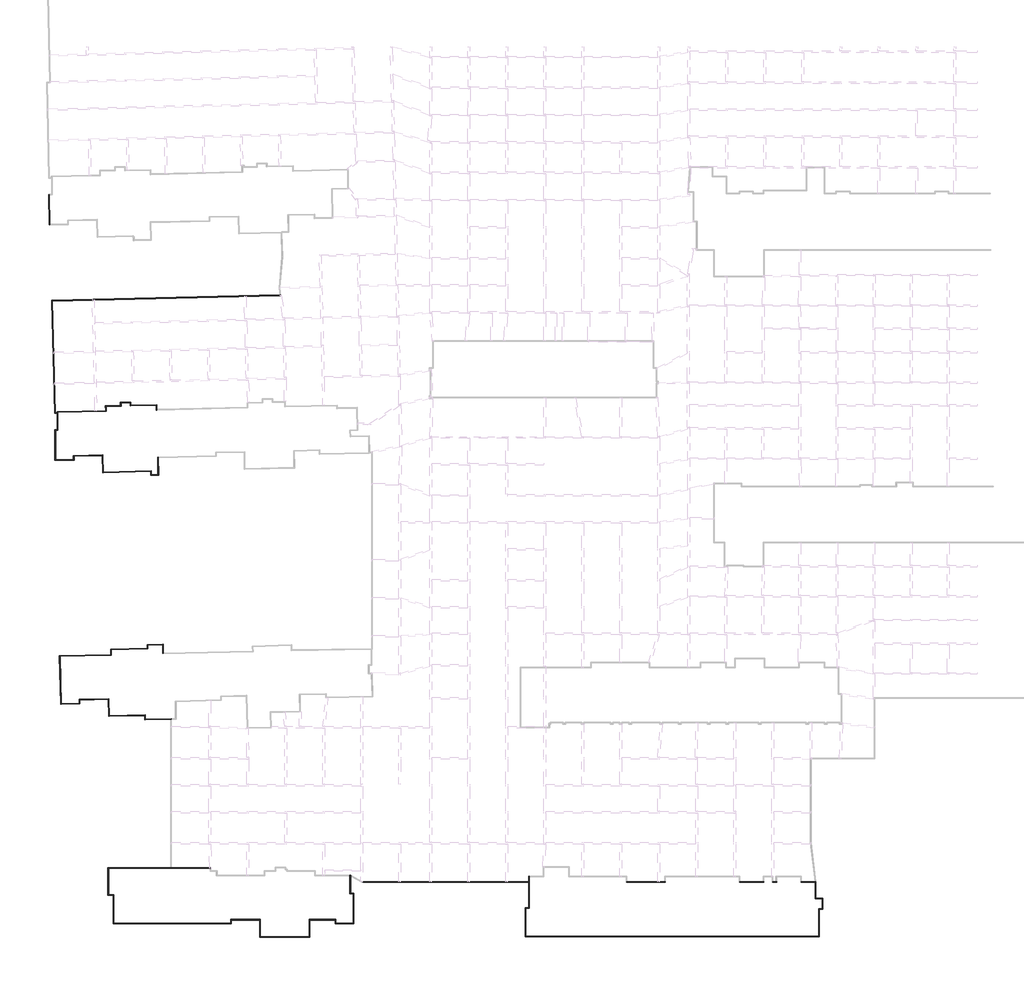
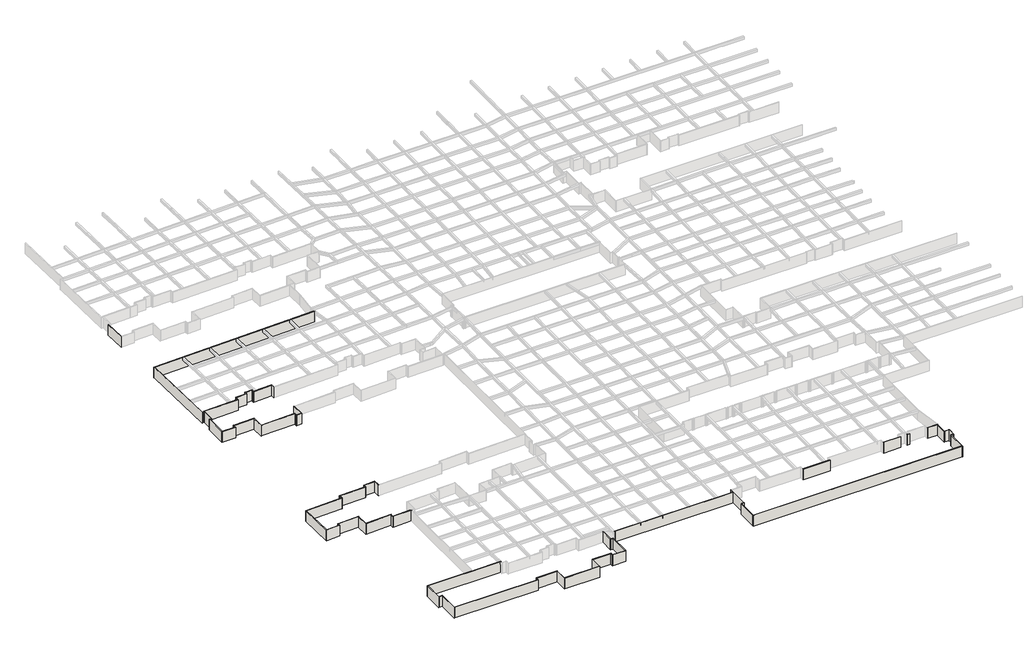
# One storey, part 1 of 20: 68 walls.
"""IFC4 building model written with IfcOpenShell, lengths in millimetres."""

from ifc_helpers import new_model, si_unit, origin, origin_with_axes, place, context, project, spatial, polyline, outline, extrude, faceted_brep, element, save

model = new_model("IFC4")

# Units and contexts
model_context = context("Model", 3, world=origin())
ifc_project = project(units=[si_unit("LENGTHUNIT", "METRE", prefix="MILLI")], contexts=[model_context])

# Site, building, storey
site = spatial("IfcSite", under=ifc_project)
building = spatial("IfcBuilding", under=site)
storey = spatial("IfcBuildingStorey", under=building, Name="户型图", Elevation=0.0)

# Walls
placement = place(None, origin())
element("IfcWall", 1, ObjectType="所有墙体", at=placement, inside=storey, context=model_context, shape_type="Brep", body=[
    faceted_brep([(-25788.9498199, 144552.0423241, 0.0), (-25635.5251271, 138236.5605216, 0.0), (-25635.5251271, 138236.5605216, 3300.0), (-25788.9498199, 144552.0423241, 3300.0), (-25668.9144149, 144552.0423241, 0.0), (-25668.9144149, 144552.0423241, 3300.0), (-25518.4748729, 138359.4394784, 3300.0), (-25515.5605216, 138239.4748729, 3300.0), (-25515.5605216, 138239.4748729, 0.0), (-25518.4748729, 138359.4394784, 0.0)], [[[0, 1, 2, 3]], [[4, 5, 6, 7, 8, 9]], [[1, 0, 4, 9, 8]], [[3, 2, 7, 6, 5]], [[0, 3, 5, 4]], [[2, 1, 8, 7]]]),
])
element("IfcWall", 2, ObjectType="所有墙体", at=placement, inside=storey, context=model_context, shape_type="Brep", body=[
    faceted_brep([(22969.277881, 123512.5246746, 0.0), (-25101.4287529, 122353.5363846, 0.0), (-25101.4287529, 122353.5363846, 3300.0), (22969.277881, 123512.5246746, 3300.0), (22986.0907128, 123392.8951605, 0.0), (22986.0907128, 123392.8951605, 3300.0), (-24978.5712471, 122236.4636154, 3300.0), (-25098.5363846, 122233.5712471, 3300.0), (-25098.5363846, 122233.5712471, 0.0), (-24978.5712471, 122236.4636154, 0.0)], [[[0, 1, 2, 3]], [[4, 5, 6, 7, 8, 9]], [[1, 0, 4, 9, 8]], [[3, 2, 7, 6, 5]], [[0, 3, 5, 4]], [[2, 1, 8, 7]]]),
])
element("IfcWall", 3, ObjectType="所有墙体", at=placement, inside=storey, context=model_context, shape_type="Brep", body=[
    faceted_brep([(-25098.5363846, 122233.5712471, 0.0), (-24529.7383934, 98641.8562998, 0.0), (-24529.7383934, 98641.8562998, 3300.0), (-25098.5363846, 122233.5712471, 3300.0), (-24978.5712471, 122236.4636154, 0.0), (-24978.5712471, 122236.4636154, 3300.0), (-24412.5967296, 98761.8562998, 3300.0), (-24409.7035208, 98641.8562998, 3300.0), (-24409.7035208, 98641.8562998, 0.0), (-24412.5967296, 98761.8562998, 0.0)], [[[0, 1, 2, 3]], [[4, 5, 6, 7, 8, 9]], [[1, 0, 4, 9, 8]], [[3, 2, 7, 6, 5]], [[0, 3, 5, 4]], [[2, 1, 8, 7]]]),
])
element("IfcWall", 4, ObjectType="所有墙体", at=placement, inside=storey, context=model_context, shape_type="SweptSolid", body=[
    extrude(outline(polyline([(-23991.1675615, 98641.8562998), (-24409.7035208, 98641.8562998), (-24412.5967296, 98761.8562998), (-23991.1675615, 98761.8562998), (-23991.1675615, 98641.8562998)])), origin_with_axes(), (0.0, 0.0, 1.0), 3300.0),
])
element("IfcWall", 5, ObjectType="所有墙体", at=placement, inside=storey, context=model_context, shape_type="Brep", body=[
    faceted_brep([(-23931.1675615, 98641.8562998, 0.0), (-23931.1675615, 95106.0245021, 0.0), (-23931.1675615, 94986.0245021, 0.0), (-23931.1675615, 94986.0245021, 3300.0), (-23931.1675615, 95106.0245021, 3300.0), (-23931.1675615, 98641.8562998, 3300.0), (-23811.1675615, 98641.8562998, 0.0), (-23811.1675615, 98641.8562998, 3300.0), (-23811.1675615, 94986.0245021, 3300.0), (-23811.1675615, 94986.0245021, 0.0)], [[[0, 1, 2, 3, 4, 5]], [[6, 7, 8, 9]], [[2, 1, 0, 6, 9]], [[5, 4, 3, 8, 7]], [[3, 2, 9, 8]], [[0, 5, 7, 6]]]),
])
element("IfcWall", 6, ObjectType="所有墙体", at=placement, inside=storey, context=model_context, shape_type="Brep", body=[
    faceted_brep([(-23931.1675615, 95106.0245021, 0.0), (-24443.0251867, 95106.0245021, 0.0), (-24443.0251867, 95106.0245021, 3300.0), (-23931.1675615, 95106.0245021, 3300.0), (-23931.1675615, 94986.0245021, 0.0), (-23931.1675615, 94986.0245021, 3300.0), (-24323.0251867, 94986.0245021, 3300.0), (-24443.0251867, 94986.0245021, 3300.0), (-24443.0251867, 94986.0245021, 0.0), (-24323.0251867, 94986.0245021, 0.0)], [[[0, 1, 2, 3]], [[4, 5, 6, 7, 8, 9]], [[1, 0, 4, 9, 8]], [[3, 2, 7, 6, 5]], [[0, 3, 5, 4]], [[2, 1, 8, 7]]]),
])
element("IfcWall", 7, ObjectType="所有墙体", at=placement, inside=storey, context=model_context, shape_type="Brep", body=[
    faceted_brep([(-24443.0251867, 94986.0245021, 0.0), (-24443.0251867, 88671.9270665, 0.0), (-24443.0251867, 88671.9270665, 3300.0), (-24443.0251867, 94986.0245021, 3300.0), (-24323.0251867, 94986.0245021, 0.0), (-24323.0251867, 94986.0245021, 3300.0), (-24323.0251867, 88791.9270665, 3300.0), (-24323.0251867, 88671.9270665, 3300.0), (-24323.0251867, 88671.9270665, 0.0), (-24323.0251867, 88791.9270665, 0.0)], [[[0, 1, 2, 3]], [[4, 5, 6, 7, 8, 9]], [[1, 0, 4, 9, 8]], [[3, 2, 7, 6, 5]], [[0, 3, 5, 4]], [[2, 1, 8, 7]]]),
])
element("IfcWall", 8, ObjectType="所有墙体", at=placement, inside=storey, context=model_context, shape_type="Brep", body=[
    faceted_brep([(-24323.0251867, 88671.9270665, 0.0), (-20418.7657678, 88671.9270665, 0.0), (-20418.7657678, 88671.9270665, 3300.0), (-24323.0251867, 88671.9270665, 3300.0), (-24323.0251867, 88791.9270665, 0.0), (-24323.0251867, 88791.9270665, 3300.0), (-20538.7657678, 88791.9270665, 3300.0), (-20418.7657678, 88791.9270665, 3300.0), (-20418.7657678, 88791.9270665, 0.0), (-20538.7657678, 88791.9270665, 0.0)], [[[0, 1, 2, 3]], [[4, 5, 6, 7, 8, 9]], [[1, 0, 4, 9, 8]], [[3, 2, 7, 6, 5]], [[0, 3, 5, 4]], [[2, 1, 8, 7]]]),
])
element("IfcWall", 9, ObjectType="所有墙体", at=placement, inside=storey, context=model_context, shape_type="Brep", body=[
    faceted_brep([(-20418.7657678, 88791.9270665, 0.0), (-20418.7657678, 89567.940823, 0.0), (-20418.7657678, 89687.9756847, 0.0), (-20418.7657678, 89687.9756847, 3300.0), (-20418.7657678, 89567.940823, 3300.0), (-20418.7657678, 88791.9270665, 3300.0), (-20538.7657678, 88791.9270665, 0.0), (-20538.7657678, 88791.9270665, 3300.0), (-20538.7657678, 89685.082933, 3300.0), (-20538.7657678, 89685.082933, 0.0)], [[[0, 1, 2, 3, 4, 5]], [[6, 7, 8, 9]], [[2, 1, 0, 6, 9]], [[5, 4, 3, 8, 7]], [[0, 5, 7, 6]], [[3, 2, 9, 8]]]),
])
element("IfcWall", 10, ObjectType="所有墙体", at=placement, inside=storey, context=model_context, shape_type="Brep", body=[
    faceted_brep([(-20418.7657678, 89567.940823, 0.0), (-14460.5366184, 89711.57147, 0.0), (-14340.57147, 89714.4633816, 0.0), (-14340.57147, 89714.4633816, 3300.0), (-14460.5366184, 89711.57147, 3300.0), (-20418.7657678, 89567.940823, 3300.0), (-20418.7657678, 89687.9756847, 0.0), (-20418.7657678, 89687.9756847, 3300.0), (-14343.4633816, 89834.42853, 3300.0), (-14343.4633816, 89834.42853, 0.0)], [[[0, 1, 2, 3, 4, 5]], [[6, 7, 8, 9]], [[2, 1, 0, 6, 9]], [[5, 4, 3, 8, 7]], [[0, 5, 7, 6]], [[3, 2, 9, 8]]]),
])
element("IfcWall", 11, ObjectType="所有墙体", at=placement, inside=storey, context=model_context, shape_type="Brep", body=[
    faceted_brep([(-14460.5366184, 89711.57147, 0.0), (-14373.7780275, 86112.5654316, 0.0), (-14373.7780275, 86112.5654316, 3300.0), (-14460.5366184, 89711.57147, 3300.0), (-14340.57147, 89714.4633816, 0.0), (-14340.57147, 89714.4633816, 3300.0), (-14256.7048016, 86235.4229484, 3300.0), (-14253.81289, 86115.4577999, 3300.0), (-14253.81289, 86115.4577999, 0.0), (-14256.7048016, 86235.4229484, 0.0)], [[[0, 1, 2, 3]], [[4, 5, 6, 7, 8, 9]], [[1, 0, 4, 9, 8]], [[3, 2, 7, 6, 5]], [[0, 3, 5, 4]], [[2, 1, 8, 7]]]),
])
element("IfcWall", 12, ObjectType="所有墙体", at=placement, inside=storey, context=model_context, shape_type="Brep", body=[
    faceted_brep([(-14253.81289, 86115.4577999, 0.0), (-4278.1756785, 86355.9711504, 0.0), (-4158.1756785, 86358.8643593, 0.0), (-4158.1756785, 86358.8643593, 3300.0), (-4278.1756785, 86355.9711504, 3300.0), (-14253.81289, 86115.4577999, 3300.0), (-14256.7048016, 86235.4229484, 0.0), (-14256.7048016, 86235.4229484, 3300.0), (-4158.1756785, 86478.899232, 3300.0), (-4158.1756785, 86478.899232, 0.0)], [[[0, 1, 2, 3, 4, 5]], [[6, 7, 8, 9]], [[2, 1, 0, 6, 9]], [[5, 4, 3, 8, 7]], [[0, 5, 7, 6]], [[3, 2, 9, 8]]]),
])
element("IfcWall", 13, ObjectType="所有墙体", at=placement, inside=storey, context=model_context, shape_type="Brep", body=[
    faceted_brep([(-4278.1756785, 86355.9711504, 0.0), (-4278.1756785, 85557.4351912, 0.0), (-4278.1756785, 85557.4351912, 3300.0), (-4278.1756785, 86355.9711504, 3300.0), (-4158.1756785, 86358.8643593, 0.0), (-4158.1756785, 86358.8643593, 3300.0), (-4158.1756785, 85677.4351912, 3300.0), (-4158.1756785, 85557.4351912, 3300.0), (-4158.1756785, 85557.4351912, 0.0), (-4158.1756785, 85677.4351912, 0.0)], [[[0, 1, 2, 3]], [[4, 5, 6, 7, 8, 9]], [[1, 0, 4, 9, 8]], [[3, 2, 7, 6, 5]], [[0, 3, 5, 4]], [[2, 1, 8, 7]]]),
])
element("IfcWall", 14, ObjectType="所有墙体", at=placement, inside=storey, context=model_context, shape_type="Brep", body=[
    faceted_brep([(-4158.1756785, 85557.4351912, 0.0), (-2635.662458, 85557.4351912, 0.0), (-2635.662458, 85557.4351912, 3300.0), (-4158.1756785, 85557.4351912, 3300.0), (-4158.1756785, 85677.4351912, 0.0), (-4158.1756785, 85677.4351912, 3300.0), (-2758.5900713, 85677.4351912, 3300.0), (-2638.5552097, 85677.4351912, 3300.0), (-2638.5552097, 85677.4351912, 0.0), (-2758.5900713, 85677.4351912, 0.0)], [[[0, 1, 2, 3]], [[4, 5, 6, 7, 8, 9]], [[1, 0, 4, 9, 8]], [[3, 2, 7, 6, 5]], [[0, 3, 5, 4]], [[2, 1, 8, 7]]]),
])
element("IfcWall", 15, ObjectType="所有墙体", at=placement, inside=storey, context=model_context, shape_type="Brep", body=[
    faceted_brep([(-2638.5552097, 85677.4351912, 0.0), (-2724.8650084, 89257.8239839, 0.0), (-2727.75692, 89377.7891324, 0.0), (-2727.75692, 89377.7891324, 3300.0), (-2724.8650084, 89257.8239839, 3300.0), (-2638.5552097, 85677.4351912, 3300.0), (-2758.5900713, 85677.4351912, 0.0), (-2758.5900713, 85677.4351912, 3300.0), (-2847.7220684, 89374.8972208, 3300.0), (-2847.7220684, 89374.8972208, 0.0)], [[[0, 1, 2, 3, 4, 5]], [[6, 7, 8, 9]], [[2, 1, 0, 6, 9]], [[5, 4, 3, 8, 7]], [[0, 5, 7, 6]], [[3, 2, 9, 8]]]),
])
element("IfcWall", 16, ObjectType="所有墙体", at=placement, inside=storey, context=model_context, shape_type="Brep", body=[
    faceted_brep([(-1631.4643758, 48099.4294775, 0.0), (-1677.2971477, 49999.433555, 0.0), (-1677.2971477, 49999.433555, 3300.0), (-1631.4643758, 48099.4294775, 3300.0), (-1751.4294775, 48096.5356242, 0.0), (-1751.4294775, 48096.5356242, 3300.0), (-1794.368396, 49876.5746, 3300.0), (-1797.2622494, 49996.5397016, 3300.0), (-1797.2622494, 49996.5397016, 0.0), (-1794.368396, 49876.5746, 0.0)], [[[0, 1, 2, 3]], [[4, 5, 6, 7, 8, 9]], [[1, 0, 4, 9, 8]], [[3, 2, 7, 6, 5]], [[0, 3, 5, 4]], [[2, 1, 8, 7]]]),
])
element("IfcWall", 17, ObjectType="所有墙体", at=placement, inside=storey, context=model_context, shape_type="Brep", body=[
    faceted_brep([(-1797.2622494, 49996.5397016, 0.0), (-4995.0208208, 49919.4018992, 0.0), (-4995.0208208, 49919.4018992, 3300.0), (-1797.2622494, 49996.5397016, 3300.0), (-1794.368396, 49876.5746, 0.0), (-1794.368396, 49876.5746, 3300.0), (-4875.0208208, 49802.2616858, 3300.0), (-4995.0208208, 49799.3669907, 3300.0), (-4995.0208208, 49799.3669907, 0.0), (-4875.0208208, 49802.2616858, 0.0)], [[[0, 1, 2, 3]], [[4, 5, 6, 7, 8, 9]], [[1, 0, 4, 9, 8]], [[3, 2, 7, 6, 5]], [[0, 3, 5, 4]], [[2, 1, 8, 7]]]),
])
element("IfcWall", 18, ObjectType="所有墙体", at=placement, inside=storey, context=model_context, shape_type="Brep", body=[
    faceted_brep([(-4995.0208208, 49799.3669907, 0.0), (-4995.0208208, 49119.4018992, 0.0), (-4995.0208208, 48999.3669907, 0.0), (-4995.0208208, 48999.3669907, 3300.0), (-4995.0208208, 49119.4018992, 3300.0), (-4995.0208208, 49799.3669907, 3300.0), (-4875.0208208, 49802.2616858, 0.0), (-4875.0208208, 49802.2616858, 3300.0), (-4875.0208208, 49002.2616858, 3300.0), (-4875.0208208, 49002.2616858, 0.0)], [[[0, 1, 2, 3, 4, 5]], [[6, 7, 8, 9]], [[2, 1, 0, 6, 9]], [[5, 4, 3, 8, 7]], [[0, 5, 7, 6]], [[3, 2, 9, 8]]]),
])
element("IfcWall", 19, ObjectType="所有墙体", at=placement, inside=storey, context=model_context, shape_type="Brep", body=[
    faceted_brep([(-4995.0208208, 49119.4018992, 0.0), (-12692.7815098, 48933.7129768, 0.0), (-12692.7815098, 48933.7129768, 3300.0), (-4995.0208208, 49119.4018992, 3300.0), (-4995.0208208, 48999.3669907, 0.0), (-4995.0208208, 48999.3669907, 3300.0), (-12572.7815098, 48816.5727634, 3300.0), (-12692.7815098, 48813.6780683, 3300.0), (-12692.7815098, 48813.6780683, 0.0), (-12572.7815098, 48816.5727634, 0.0)], [[[0, 1, 2, 3]], [[4, 5, 6, 7, 8, 9]], [[1, 0, 4, 9, 8]], [[3, 2, 7, 6, 5]], [[0, 3, 5, 4]], [[2, 1, 8, 7]]]),
])
element("IfcWall", 20, ObjectType="所有墙体", at=placement, inside=storey, context=model_context, shape_type="Brep", body=[
    faceted_brep([(-12692.7815098, 48813.6780683, 0.0), (-12692.7815098, 47833.7129768, 0.0), (-12692.7815098, 47713.6780683, 0.0), (-12692.7815098, 47713.6780683, 3300.0), (-12692.7815098, 47833.7129768, 3300.0), (-12692.7815098, 48813.6780683, 3300.0), (-12572.7815098, 48816.5727634, 0.0), (-12572.7815098, 48816.5727634, 3300.0), (-12572.7815098, 47716.5727634, 3300.0), (-12572.7815098, 47716.5727634, 0.0)], [[[0, 1, 2, 3, 4, 5]], [[6, 7, 8, 9]], [[2, 1, 0, 6, 9]], [[5, 4, 3, 8, 7]], [[0, 5, 7, 6]], [[3, 2, 9, 8]]]),
])
element("IfcWall", 21, ObjectType="所有墙体", at=placement, inside=storey, context=model_context, shape_type="Brep", body=[
    faceted_brep([(-12692.7815098, 47833.7129768, 0.0), (-23491.0701354, 47573.231694, 0.0), (-23491.0701354, 47573.231694, 3300.0), (-12692.7815098, 47833.7129768, 3300.0), (-12692.7815098, 47713.6780683, 0.0), (-12692.7815098, 47713.6780683, 3300.0), (-23368.2111804, 47456.1604457, 3300.0), (-23488.176282, 47453.2665924, 3300.0), (-23488.176282, 47453.2665924, 0.0), (-23368.2111804, 47456.1604457, 0.0)], [[[0, 1, 2, 3]], [[4, 5, 6, 7, 8, 9]], [[1, 0, 4, 9, 8]], [[3, 2, 7, 6, 5]], [[0, 3, 5, 4]], [[2, 1, 8, 7]]]),
])
element("IfcWall", 22, ObjectType="所有墙体", at=placement, inside=storey, context=model_context, shape_type="Brep", body=[
    faceted_brep([(-23488.176282, 47453.2665924, 0.0), (-23244.6102929, 37356.2038705, 0.0), (-23244.6102929, 37356.2038705, 3300.0), (-23488.176282, 47453.2665924, 3300.0), (-23368.2111804, 47456.1604457, 0.0), (-23368.2111804, 47456.1604457, 3300.0), (-23127.5390446, 37479.0628255, 3300.0), (-23124.6451913, 37359.0977239, 3300.0), (-23124.6451913, 37359.0977239, 0.0), (-23127.5390446, 37479.0628255, 0.0)], [[[0, 1, 2, 3]], [[4, 5, 6, 7, 8, 9]], [[1, 0, 4, 9, 8]], [[3, 2, 7, 6, 5]], [[0, 3, 5, 4]], [[2, 1, 8, 7]]]),
])
element("IfcWall", 23, ObjectType="所有墙体", at=placement, inside=storey, context=model_context, shape_type="Brep", body=[
    faceted_brep([(-23124.6451913, 37359.0977239, 0.0), (-19181.0199443, 37454.2276652, 0.0), (-19181.0199443, 37454.2276652, 3300.0), (-23124.6451913, 37359.0977239, 3300.0), (-23127.5390446, 37479.0628255, 0.0), (-23127.5390446, 37479.0628255, 3300.0), (-19301.0199443, 37571.3678785, 3300.0), (-19181.0199443, 37574.2625737, 3300.0), (-19181.0199443, 37574.2625737, 0.0), (-19301.0199443, 37571.3678785, 0.0)], [[[0, 1, 2, 3]], [[4, 5, 6, 7, 8, 9]], [[1, 0, 4, 9, 8]], [[3, 2, 7, 6, 5]], [[0, 3, 5, 4]], [[2, 1, 8, 7]]]),
])
element("IfcWall", 24, ObjectType="所有墙体", at=placement, inside=storey, context=model_context, shape_type="Brep", body=[
    faceted_brep([(-19181.0199443, 37574.2625737, 0.0), (-19181.0199443, 38254.2276652, 0.0), (-19181.0199443, 38374.2625737, 0.0), (-19181.0199443, 38374.2625737, 3300.0), (-19181.0199443, 38254.2276652, 3300.0), (-19181.0199443, 37574.2625737, 3300.0), (-19301.0199443, 37571.3678785, 0.0), (-19301.0199443, 37571.3678785, 3300.0), (-19301.0199443, 38371.3678785, 3300.0), (-19301.0199443, 38371.3678785, 0.0)], [[[0, 1, 2, 3, 4, 5]], [[6, 7, 8, 9]], [[2, 1, 0, 6, 9]], [[5, 4, 3, 8, 7]], [[0, 5, 7, 6]], [[3, 2, 9, 8]]]),
])
element("IfcWall", 25, ObjectType="所有墙体", at=placement, inside=storey, context=model_context, shape_type="Brep", body=[
    faceted_brep([(-19181.0199443, 38254.2276652, 0.0), (-13201.3295681, 38398.4725056, 0.0), (-13081.3644665, 38401.3663589, 0.0), (-13081.3644665, 38401.3663589, 3300.0), (-13201.3295681, 38398.4725056, 3300.0), (-19181.0199443, 38254.2276652, 3300.0), (-19181.0199443, 38374.2625737, 0.0), (-19181.0199443, 38374.2625737, 3300.0), (-13084.2583198, 38521.3314606, 3300.0), (-13084.2583198, 38521.3314606, 0.0)], [[[0, 1, 2, 3, 4, 5]], [[6, 7, 8, 9]], [[2, 1, 0, 6, 9]], [[5, 4, 3, 8, 7]], [[0, 5, 7, 6]], [[3, 2, 9, 8]]]),
])
element("IfcWall", 26, ObjectType="所有墙体", at=placement, inside=storey, context=model_context, shape_type="Brep", body=[
    faceted_brep([(-13201.3295681, 38398.4725056, 0.0), (-13114.5027165, 34799.0530208, 0.0), (-13114.5027165, 34799.0530208, 3300.0), (-13201.3295681, 38398.4725056, 3300.0), (-13081.3644665, 38401.3663589, 0.0), (-13081.3644665, 38401.3663589, 3300.0), (-12997.4314682, 34921.9119758, 3300.0), (-12994.5376148, 34801.9468741, 3300.0), (-12994.5376148, 34801.9468741, 0.0), (-12997.4314682, 34921.9119758, 0.0)], [[[0, 1, 2, 3]], [[4, 5, 6, 7, 8, 9]], [[1, 0, 4, 9, 8]], [[3, 2, 7, 6, 5]], [[0, 3, 5, 4]], [[2, 1, 8, 7]]]),
])
element("IfcWall", 27, ObjectType="所有墙体", at=placement, inside=storey, context=model_context, shape_type="Brep", body=[
    faceted_brep([(-12994.5376148, 34801.9468741, 0.0), (-5538.0068821, 34981.8167366, 0.0), (-5418.0068821, 34984.7114318, 0.0), (-5418.0068821, 34984.7114318, 3300.0), (-5538.0068821, 34981.8167366, 3300.0), (-12994.5376148, 34801.9468741, 3300.0), (-12997.4314682, 34921.9119758, 0.0), (-12997.4314682, 34921.9119758, 3300.0), (-5418.0068821, 35104.7463403, 3300.0), (-5418.0068821, 35104.7463403, 0.0)], [[[0, 1, 2, 3, 4, 5]], [[6, 7, 8, 9]], [[2, 1, 0, 6, 9]], [[5, 4, 3, 8, 7]], [[0, 5, 7, 6]], [[3, 2, 9, 8]]]),
])
element("IfcWall", 28, ObjectType="所有墙体", at=placement, inside=storey, context=model_context, shape_type="Brep", body=[
    faceted_brep([(-5538.0068821, 34981.8167366, 0.0), (-5538.0068821, 34081.8167366, 0.0), (-5538.0068821, 34081.8167366, 3300.0), (-5538.0068821, 34981.8167366, 3300.0), (-5418.0068821, 34984.7114318, 0.0), (-5418.0068821, 34984.7114318, 3300.0), (-5418.0068821, 34204.7463403, 3300.0), (-5418.0068821, 34084.7114318, 3300.0), (-5418.0068821, 34084.7114318, 0.0), (-5418.0068821, 34204.7463403, 0.0)], [[[0, 1, 2, 3]], [[4, 5, 6, 7, 8, 9]], [[1, 0, 4, 9, 8]], [[3, 2, 7, 6, 5]], [[0, 3, 5, 4]], [[2, 1, 8, 7]]]),
])
element("IfcWall", 29, ObjectType="所有墙体", at=placement, inside=storey, context=model_context, shape_type="Brep", body=[
    faceted_brep([(-5418.0068821, 34084.7114318, 0.0), (-39.60639, 34214.4516812, 0.0), (80.39361, 34217.3463764, 0.0), (80.39361, 34217.3463764, 3300.0), (-39.60639, 34214.4516812, 3300.0), (-5418.0068821, 34084.7114318, 3300.0), (-5418.0068821, 34204.7463403, 0.0), (-5418.0068821, 34204.7463403, 3300.0), (-15.923934, 34335.0578688, 3300.0), (80.39361, 34337.3812849, 3300.0), (80.39361, 34337.3812849, 0.0), (-15.923934, 34335.0578688, 0.0), (80.39361, 34226.3096315, 0.0), (80.39361, 34226.3096315, 3300.0)], [[[0, 1, 2, 3, 4, 5]], [[6, 7, 8, 9, 10, 11]], [[2, 1, 0, 6, 11, 10, 12]], [[5, 4, 3, 13, 9, 8, 7]], [[0, 5, 7, 6]], [[3, 2, 12, 10, 9, 13]]]),
])
element("IfcWall", 30, ObjectType="所有墙体", at=placement, inside=storey, context=model_context, shape_type="Brep", body=[
    faceted_brep([(8377.0, 2935.916483, 0.0), (80.39361, 2935.916483, 0.0), (-39.60639, 2935.916483, 0.0), (-13291.0, 2935.916483, 0.0), (-13291.0, 2935.916483, 3300.0), (-39.60639, 2935.916483, 3300.0), (80.39361, 2935.916483, 3300.0), (8377.0, 2935.916483, 3300.0), (8377.0, 2815.916483, 0.0), (8377.0, 2815.916483, 3300.0), (8257.0, 2815.916483, 3300.0), (-13171.0, 2815.916483, 3300.0), (-13291.0, 2815.916483, 3300.0), (-13291.0, 2815.916483, 0.0), (-13171.0, 2815.916483, 0.0), (8257.0, 2815.916483, 0.0)], [[[0, 1, 2, 3, 4, 5, 6, 7]], [[8, 9, 10, 11, 12, 13, 14, 15]], [[3, 2, 1, 0, 8, 15, 14, 13]], [[7, 6, 5, 4, 12, 11, 10, 9]], [[4, 3, 13, 12]], [[0, 7, 9, 8]]]),
])
element("IfcWall", 31, ObjectType="所有墙体", at=placement, inside=storey, context=model_context, shape_type="Brep", body=[
    faceted_brep([(-13291.0, 2815.916483, 0.0), (-13291.0, -2803.0, 0.0), (-13291.0, -2803.0, 3300.0), (-13291.0, 2815.916483, 3300.0), (-13171.0, 2815.916483, 0.0), (-13171.0, 2815.916483, 3300.0), (-13171.0, -2683.0, 3300.0), (-13171.0, -2803.0, 3300.0), (-13171.0, -2803.0, 0.0), (-13171.0, -2683.0, 0.0)], [[[0, 1, 2, 3]], [[4, 5, 6, 7, 8, 9]], [[1, 0, 4, 9, 8]], [[3, 2, 7, 6, 5]], [[0, 3, 5, 4]], [[2, 1, 8, 7]]]),
])
element("IfcWall", 32, ObjectType="所有墙体", at=placement, inside=storey, context=model_context, shape_type="Brep", body=[
    faceted_brep([(-13171.0, -2803.0, 0.0), (-12208.8785992, -2803.0, 0.0), (-12088.8785992, -2803.0, 0.0), (-12088.8785992, -2803.0, 3300.0), (-12208.8785992, -2803.0, 3300.0), (-13171.0, -2803.0, 3300.0), (-13171.0, -2683.0, 0.0), (-13171.0, -2683.0, 3300.0), (-12088.8785992, -2683.0, 3300.0), (-12088.8785992, -2683.0, 0.0)], [[[0, 1, 2, 3, 4, 5]], [[6, 7, 8, 9]], [[2, 1, 0, 6, 9]], [[5, 4, 3, 8, 7]], [[0, 5, 7, 6]], [[3, 2, 9, 8]]]),
])
element("IfcWall", 33, ObjectType="所有墙体", at=placement, inside=storey, context=model_context, shape_type="Brep", body=[
    faceted_brep([(-12208.8785992, -2803.0, 0.0), (-12208.8785992, -8850.0, 0.0), (-12208.8785992, -8850.0, 3300.0), (-12208.8785992, -2803.0, 3300.0), (-12088.8785992, -2803.0, 0.0), (-12088.8785992, -2803.0, 3300.0), (-12088.8785992, -8730.0, 3300.0), (-12088.8785992, -8850.0, 3300.0), (-12088.8785992, -8850.0, 0.0), (-12088.8785992, -8730.0, 0.0)], [[[0, 1, 2, 3]], [[4, 5, 6, 7, 8, 9]], [[1, 0, 4, 9, 8]], [[3, 2, 7, 6, 5]], [[0, 3, 5, 4]], [[2, 1, 8, 7]]]),
])
element("IfcWall", 34, ObjectType="所有墙体", at=placement, inside=storey, context=model_context, shape_type="Brep", body=[
    faceted_brep([(-12088.8785992, -8850.0, 0.0), (12627.0, -8850.0, 0.0), (12627.0, -8850.0, 3300.0), (-12088.8785992, -8850.0, 3300.0), (-12088.8785992, -8730.0, 0.0), (-12088.8785992, -8730.0, 3300.0), (12507.0, -8730.0, 3300.0), (12627.0, -8730.0, 3300.0), (12627.0, -8730.0, 0.0), (12507.0, -8730.0, 0.0)], [[[0, 1, 2, 3]], [[4, 5, 6, 7, 8, 9]], [[1, 0, 4, 9, 8]], [[3, 2, 7, 6, 5]], [[0, 3, 5, 4]], [[2, 1, 8, 7]]]),
])
element("IfcWall", 35, ObjectType="所有墙体", at=placement, inside=storey, context=model_context, shape_type="Brep", body=[
    faceted_brep([(12627.0, -8730.0, 0.0), (12627.0, -8053.0, 0.0), (12627.0, -7933.0, 0.0), (12627.0, -7933.0, 3300.0), (12627.0, -8053.0, 3300.0), (12627.0, -8730.0, 3300.0), (12507.0, -8730.0, 0.0), (12507.0, -8730.0, 3300.0), (12507.0, -7933.0, 3300.0), (12507.0, -7933.0, 0.0)], [[[0, 1, 2, 3, 4, 5]], [[6, 7, 8, 9]], [[2, 1, 0, 6, 9]], [[5, 4, 3, 8, 7]], [[0, 5, 7, 6]], [[3, 2, 9, 8]]]),
])
element("IfcWall", 36, ObjectType="所有墙体", at=placement, inside=storey, context=model_context, shape_type="Brep", body=[
    faceted_brep([(12627.0, -8053.0, 0.0), (18657.0, -8053.0, 0.0), (18777.0, -8053.0, 0.0), (18777.0, -8053.0, 3300.0), (18657.0, -8053.0, 3300.0), (12627.0, -8053.0, 3300.0), (12627.0, -7933.0, 0.0), (12627.0, -7933.0, 3300.0), (18777.0, -7933.0, 3300.0), (18777.0, -7933.0, 0.0)], [[[0, 1, 2, 3, 4, 5]], [[6, 7, 8, 9]], [[2, 1, 0, 6, 9]], [[5, 4, 3, 8, 7]], [[0, 5, 7, 6]], [[3, 2, 9, 8]]]),
])
element("IfcWall", 37, ObjectType="所有墙体", at=placement, inside=storey, context=model_context, shape_type="Brep", body=[
    faceted_brep([(18657.0, -8053.0, 0.0), (18657.0, -11652.0, 0.0), (18657.0, -11652.0, 3300.0), (18657.0, -8053.0, 3300.0), (18777.0, -8053.0, 0.0), (18777.0, -8053.0, 3300.0), (18777.0, -11532.0, 3300.0), (18777.0, -11652.0, 3300.0), (18777.0, -11652.0, 0.0), (18777.0, -11532.0, 0.0)], [[[0, 1, 2, 3]], [[4, 5, 6, 7, 8, 9]], [[1, 0, 4, 9, 8]], [[3, 2, 7, 6, 5]], [[0, 3, 5, 4]], [[2, 1, 8, 7]]]),
])
element("IfcWall", 38, ObjectType="所有墙体", at=placement, inside=storey, context=model_context, shape_type="Brep", body=[
    faceted_brep([(18777.0, -11652.0, 0.0), (29176.0, -11652.0, 0.0), (29176.0, -11652.0, 3300.0), (18777.0, -11652.0, 3300.0), (18777.0, -11532.0, 0.0), (18777.0, -11532.0, 3300.0), (29056.0, -11532.0, 3300.0), (29176.0, -11532.0, 3300.0), (29176.0, -11532.0, 0.0), (29056.0, -11532.0, 0.0)], [[[0, 1, 2, 3]], [[4, 5, 6, 7, 8, 9]], [[1, 0, 4, 9, 8]], [[3, 2, 7, 6, 5]], [[0, 3, 5, 4]], [[2, 1, 8, 7]]]),
])
element("IfcWall", 39, ObjectType="所有墙体", at=placement, inside=storey, context=model_context, shape_type="Brep", body=[
    faceted_brep([(29176.0, -11532.0, 0.0), (29176.0, -8053.0, 0.0), (29176.0, -7933.0, 0.0), (29176.0, -7933.0, 3300.0), (29176.0, -8053.0, 3300.0), (29176.0, -11532.0, 3300.0), (29056.0, -11532.0, 0.0), (29056.0, -11532.0, 3300.0), (29056.0, -7933.0, 3300.0), (29056.0, -7933.0, 0.0)], [[[0, 1, 2, 3, 4, 5]], [[6, 7, 8, 9]], [[2, 1, 0, 6, 9]], [[5, 4, 3, 8, 7]], [[0, 5, 7, 6]], [[3, 2, 9, 8]]]),
])
element("IfcWall", 40, ObjectType="所有墙体", at=placement, inside=storey, context=model_context, shape_type="Brep", body=[
    faceted_brep([(29176.0, -8053.0, 0.0), (34506.0, -8053.0, 0.0), (34626.0, -8053.0, 0.0), (34626.0, -8053.0, 3300.0), (34506.0, -8053.0, 3300.0), (29176.0, -8053.0, 3300.0), (29176.0, -7933.0, 0.0), (29176.0, -7933.0, 3300.0), (34626.0, -7933.0, 3300.0), (34626.0, -7933.0, 0.0)], [[[0, 1, 2, 3, 4, 5]], [[6, 7, 8, 9]], [[2, 1, 0, 6, 9]], [[5, 4, 3, 8, 7]], [[0, 5, 7, 6]], [[3, 2, 9, 8]]]),
])
element("IfcWall", 41, ObjectType="所有墙体", at=placement, inside=storey, context=model_context, shape_type="Brep", body=[
    faceted_brep([(34506.0, -8053.0, 0.0), (34506.0, -8850.0, 0.0), (34506.0, -8850.0, 3300.0), (34506.0, -8053.0, 3300.0), (34626.0, -8053.0, 0.0), (34626.0, -8053.0, 3300.0), (34626.0, -8730.0, 3300.0), (34626.0, -8850.0, 3300.0), (34626.0, -8850.0, 0.0), (34626.0, -8730.0, 0.0)], [[[0, 1, 2, 3]], [[4, 5, 6, 7, 8, 9]], [[1, 0, 4, 9, 8]], [[3, 2, 7, 6, 5]], [[0, 3, 5, 4]], [[2, 1, 8, 7]]]),
])
element("IfcWall", 42, ObjectType="所有墙体", at=placement, inside=storey, context=model_context, shape_type="Brep", body=[
    faceted_brep([(34626.0, -8850.0, 0.0), (38475.0, -8850.0, 0.0), (38475.0, -8850.0, 3300.0), (34626.0, -8850.0, 3300.0), (34626.0, -8730.0, 0.0), (34626.0, -8730.0, 3300.0), (38355.0, -8730.0, 3300.0), (38475.0, -8730.0, 3300.0), (38475.0, -8730.0, 0.0), (38355.0, -8730.0, 0.0)], [[[0, 1, 2, 3]], [[4, 5, 6, 7, 8, 9]], [[1, 0, 4, 9, 8]], [[3, 2, 7, 6, 5]], [[0, 3, 5, 4]], [[2, 1, 8, 7]]]),
])
element("IfcWall", 43, ObjectType="所有墙体", at=placement, inside=storey, context=model_context, shape_type="Brep", body=[
    faceted_brep([(38475.0, -8730.0, 0.0), (38475.0, -2429.0, 0.0), (38475.0, -2429.0, 3300.0), (38475.0, -8730.0, 3300.0), (38355.0, -8730.0, 0.0), (38355.0, -8730.0, 3300.0), (38355.0, -2549.0, 3300.0), (38355.0, -2429.0, 3300.0), (38355.0, -2429.0, 0.0), (38355.0, -2549.0, 0.0)], [[[0, 1, 2, 3]], [[4, 5, 6, 7, 8, 9]], [[1, 0, 4, 9, 8]], [[3, 2, 7, 6, 5]], [[0, 3, 5, 4]], [[2, 1, 8, 7]]]),
])
element("IfcWall", 44, ObjectType="所有墙体", at=placement, inside=storey, context=model_context, shape_type="Brep", body=[
    faceted_brep([(38355.0, -2429.0, 0.0), (37775.0, -2429.0, 0.0), (37655.0, -2429.0, 0.0), (37655.0, -2429.0, 3300.0), (37775.0, -2429.0, 3300.0), (38355.0, -2429.0, 3300.0), (38355.0, -2549.0, 0.0), (38355.0, -2549.0, 3300.0), (37655.0, -2549.0, 3300.0), (37655.0, -2549.0, 0.0)], [[[0, 1, 2, 3, 4, 5]], [[6, 7, 8, 9]], [[2, 1, 0, 6, 9]], [[5, 4, 3, 8, 7]], [[0, 5, 7, 6]], [[3, 2, 9, 8]]]),
])
element("IfcWall", 45, ObjectType="所有墙体", at=placement, inside=storey, context=model_context, shape_type="Brep", body=[
    faceted_brep([(37775.0, -2429.0, 0.0), (37775.0, 1211.1432311, 0.0), (37775.0, 1347.0516371, 0.0), (37775.0, 1347.0516371, 3300.0), (37775.0, 1211.1432311, 3300.0), (37775.0, -2429.0, 3300.0), (37655.0, -2429.0, 0.0), (37655.0, -2429.0, 3300.0), (37655.0, 1251.0, 3300.0), (37655.0, 1371.0, 3300.0), (37655.0, 1410.8567689, 3300.0), (37655.0, 1410.8567689, 0.0), (37655.0, 1371.0, 0.0), (37655.0, 1251.0, 0.0)], [[[0, 1, 2, 3, 4, 5]], [[6, 7, 8, 9, 10, 11, 12, 13]], [[2, 1, 0, 6, 13, 12, 11]], [[5, 4, 3, 10, 9, 8, 7]], [[0, 5, 7, 6]], [[3, 2, 11, 10]]]),
])
element("IfcWall", 46, ObjectType="所有墙体", at=placement, inside=storey, context=model_context, shape_type="SweptSolid", body=[
    extrude(outline(polyline([(75227.25326, -63.5203758), (40427.900116, -63.5203758), (40202.2129402, 56.4796242), (75227.25326, 56.4796242), (75227.25326, -63.5203758)])), origin_with_axes(), (0.0, 0.0, 1.0), 3300.0),
])
element("IfcWall", 47, ObjectType="所有墙体", at=placement, inside=storey, context=model_context, shape_type="Brep", body=[
    faceted_brep([(75347.25326, -5434.0, 0.0), (75347.25326, 1046.0, 0.0), (75347.25326, 1166.0, 0.0), (75347.25326, 1166.0, 3300.0), (75347.25326, 1046.0, 3300.0), (75347.25326, -5434.0, 3300.0), (75227.25326, -5434.0, 0.0), (75227.25326, -5434.0, 3300.0), (75227.25326, -63.5203758, 3300.0), (75227.25326, 56.4796242, 3300.0), (75227.25326, 1166.0, 3300.0), (75227.25326, 1166.0, 0.0), (75227.25326, 56.4796242, 0.0), (75227.25326, -63.5203758, 0.0)], [[[0, 1, 2, 3, 4, 5]], [[6, 7, 8, 9, 10, 11, 12, 13]], [[2, 1, 0, 6, 13, 12, 11]], [[5, 4, 3, 10, 9, 8, 7]], [[3, 2, 11, 10]], [[0, 5, 7, 6]]]),
])
element("IfcWall", 48, ObjectType="所有墙体", at=placement, inside=storey, context=model_context, shape_type="Brep", body=[
    faceted_brep([(95932.0, -63.5203758, 0.0), (103982.0, -63.5203758, 0.0), (103982.0, -63.5203758, 3300.0), (95932.0, -63.5203758, 3300.0), (95932.0, 56.4796242, 0.0), (95932.0, 56.4796242, 3300.0), (103862.0, 56.4796242, 3300.0), (103982.0, 56.4796242, 3300.0), (103982.0, 56.4796242, 0.0), (103862.0, 56.4796242, 0.0)], [[[0, 1, 2, 3]], [[4, 5, 6, 7, 8, 9]], [[1, 0, 4, 9, 8]], [[3, 2, 7, 6, 5]], [[0, 3, 5, 4]], [[2, 1, 8, 7]]]),
])
element("IfcWall", 49, ObjectType="所有墙体", at=placement, inside=storey, context=model_context, shape_type="Brep", body=[
    faceted_brep([(119682.0, -63.5203758, 0.0), (124732.0, -63.5203758, 0.0), (124732.0, -63.5203758, 3300.0), (119682.0, -63.5203758, 3300.0), (119682.0, 56.4796242, 0.0), (119682.0, 56.4796242, 3300.0), (124612.0, 56.4796242, 3300.0), (124732.0, 56.4796242, 3300.0), (124732.0, 56.4796242, 0.0), (124612.0, 56.4796242, 0.0)], [[[0, 1, 2, 3]], [[4, 5, 6, 7, 8, 9]], [[1, 0, 4, 9, 8]], [[3, 2, 7, 6, 5]], [[0, 3, 5, 4]], [[2, 1, 8, 7]]]),
])
element("IfcWall", 50, ObjectType="所有墙体", at=placement, inside=storey, context=model_context, shape_type="Brep", body=[
    faceted_brep([(126632.0, -63.5203758, 0.0), (127432.0, -63.5203758, 0.0), (127432.0, -63.5203758, 3300.0), (126632.0, -63.5203758, 3300.0), (126632.0, 56.4796242, 0.0), (126632.0, 56.4796242, 3300.0), (127312.0, 56.4796242, 3300.0), (127432.0, 56.4796242, 3300.0), (127432.0, 56.4796242, 0.0), (127312.0, 56.4796242, 0.0)], [[[0, 1, 2, 3]], [[4, 5, 6, 7, 8, 9]], [[1, 0, 4, 9, 8]], [[3, 2, 7, 6, 5]], [[0, 3, 5, 4]], [[2, 1, 8, 7]]]),
])
element("IfcWall", 51, ObjectType="所有墙体", at=placement, inside=storey, context=model_context, shape_type="Brep", body=[
    faceted_brep([(132682.0, -63.5203758, 0.0), (135575.2504114, -63.5203758, 0.0), (135695.2504114, -63.5203758, 0.0), (135695.2504114, -63.5203758, 3300.0), (135575.2504114, -63.5203758, 3300.0), (132682.0, -63.5203758, 3300.0), (132682.0, 56.4796242, 0.0), (132682.0, 56.4796242, 3300.0), (135567.4327482, 56.4796242, 3300.0), (135688.3339273, 56.4796242, 3300.0), (135695.2504114, 56.4796242, 3300.0), (135695.2504114, 56.4796242, 0.0), (135688.3339273, 56.4796242, 0.0), (135567.4327482, 56.4796242, 0.0)], [[[0, 1, 2, 3, 4, 5]], [[6, 7, 8, 9, 10, 11, 12, 13]], [[2, 1, 0, 6, 13, 12, 11]], [[5, 4, 3, 10, 9, 8, 7]], [[0, 5, 7, 6]], [[3, 2, 11, 10]]]),
])
element("IfcWall", 52, ObjectType="所有墙体", at=placement, inside=storey, context=model_context, shape_type="Brep", body=[
    faceted_brep([(135575.2504114, -63.5203758, 0.0), (135575.2504114, -3604.0, 0.0), (135575.2504114, -3604.0, 3300.0), (135575.2504114, -63.5203758, 3300.0), (135695.2504114, -63.5203758, 0.0), (135695.2504114, -63.5203758, 3300.0), (135695.2504114, -3484.0, 3300.0), (135695.2504114, -3604.0, 3300.0), (135695.2504114, -3604.0, 0.0), (135695.2504114, -3484.0, 0.0)], [[[0, 1, 2, 3]], [[4, 5, 6, 7, 8, 9]], [[1, 0, 4, 9, 8]], [[3, 2, 7, 6, 5]], [[0, 3, 5, 4]], [[2, 1, 8, 7]]]),
])
element("IfcWall", 53, ObjectType="所有墙体", at=placement, inside=storey, context=model_context, shape_type="Brep", body=[
    faceted_brep([(135695.2504114, -3604.0, 0.0), (137012.0, -3604.0, 0.0), (137132.0, -3604.0, 0.0), (137132.0, -3604.0, 3300.0), (137012.0, -3604.0, 3300.0), (135695.2504114, -3604.0, 3300.0), (135695.2504114, -3484.0, 0.0), (135695.2504114, -3484.0, 3300.0), (137132.0, -3484.0, 3300.0), (137132.0, -3484.0, 0.0)], [[[0, 1, 2, 3, 4, 5]], [[6, 7, 8, 9]], [[2, 1, 0, 6, 9]], [[5, 4, 3, 8, 7]], [[0, 5, 7, 6]], [[3, 2, 9, 8]]]),
])
element("IfcWall", 54, ObjectType="所有墙体", at=placement, inside=storey, context=model_context, shape_type="Brep", body=[
    faceted_brep([(137012.0, -3604.0, 0.0), (137012.0, -5684.0, 0.0), (137012.0, -5804.0, 0.0), (137012.0, -5804.0, 3300.0), (137012.0, -5684.0, 3300.0), (137012.0, -3604.0, 3300.0), (137132.0, -3604.0, 0.0), (137132.0, -3604.0, 3300.0), (137132.0, -5804.0, 3300.0), (137132.0, -5804.0, 0.0)], [[[0, 1, 2, 3, 4, 5]], [[6, 7, 8, 9]], [[2, 1, 0, 6, 9]], [[5, 4, 3, 8, 7]], [[0, 5, 7, 6]], [[3, 2, 9, 8]]]),
])
element("IfcWall", 55, ObjectType="所有墙体", at=placement, inside=storey, context=model_context, shape_type="Brep", body=[
    faceted_brep([(137012.0, -5684.0, 0.0), (136262.0, -5684.0, 0.0), (136262.0, -5684.0, 3300.0), (137012.0, -5684.0, 3300.0), (137012.0, -5804.0, 0.0), (137012.0, -5804.0, 3300.0), (136382.0, -5804.0, 3300.0), (136262.0, -5804.0, 3300.0), (136262.0, -5804.0, 0.0), (136382.0, -5804.0, 0.0)], [[[0, 1, 2, 3]], [[4, 5, 6, 7, 8, 9]], [[1, 0, 4, 9, 8]], [[3, 2, 7, 6, 5]], [[0, 3, 5, 4]], [[2, 1, 8, 7]]]),
])
element("IfcWall", 56, ObjectType="所有墙体", at=placement, inside=storey, context=model_context, shape_type="Brep", body=[
    faceted_brep([(136262.0, -5804.0, 0.0), (136262.0, -11434.0, 0.0), (136262.0, -11554.0, 0.0), (136262.0, -11554.0, 3300.0), (136262.0, -11434.0, 3300.0), (136262.0, -5804.0, 3300.0), (136382.0, -5804.0, 0.0), (136382.0, -5804.0, 3300.0), (136382.0, -11554.0, 3300.0), (136382.0, -11554.0, 0.0)], [[[0, 1, 2, 3, 4, 5]], [[6, 7, 8, 9]], [[2, 1, 0, 6, 9]], [[5, 4, 3, 8, 7]], [[0, 5, 7, 6]], [[3, 2, 9, 8]]]),
])
element("IfcWall", 57, ObjectType="所有墙体", at=placement, inside=storey, context=model_context, shape_type="Brep", body=[
    faceted_brep([(136262.0, -11434.0, 0.0), (74632.0, -11434.0, 0.0), (74512.0, -11434.0, 0.0), (74512.0, -11434.0, 3300.0), (74632.0, -11434.0, 3300.0), (136262.0, -11434.0, 3300.0), (136262.0, -11554.0, 0.0), (136262.0, -11554.0, 3300.0), (74512.0, -11554.0, 3300.0), (74512.0, -11554.0, 0.0)], [[[0, 1, 2, 3, 4, 5]], [[6, 7, 8, 9]], [[2, 1, 0, 6, 9]], [[5, 4, 3, 8, 7]], [[0, 5, 7, 6]], [[3, 2, 9, 8]]]),
])
element("IfcWall", 58, ObjectType="所有墙体", at=placement, inside=storey, context=model_context, shape_type="Brep", body=[
    faceted_brep([(74632.0, -11434.0, 0.0), (74632.0, -5554.0, 0.0), (74632.0, -5434.0, 0.0), (74632.0, -5434.0, 3300.0), (74632.0, -5554.0, 3300.0), (74632.0, -11434.0, 3300.0), (74512.0, -11434.0, 0.0), (74512.0, -11434.0, 3300.0), (74512.0, -5434.0, 3300.0), (74512.0, -5434.0, 0.0)], [[[0, 1, 2, 3, 4, 5]], [[6, 7, 8, 9]], [[2, 1, 0, 6, 9]], [[5, 4, 3, 8, 7]], [[0, 5, 7, 6]], [[3, 2, 9, 8]]]),
])
element("IfcWall", 59, ObjectType="所有墙体", at=placement, inside=storey, context=model_context, shape_type="Brep", body=[
    faceted_brep([(74632.0, -5554.0, 0.0), (75347.25326, -5554.0, 0.0), (75347.25326, -5554.0, 3300.0), (74632.0, -5554.0, 3300.0), (74632.0, -5434.0, 0.0), (74632.0, -5434.0, 3300.0), (75227.25326, -5434.0, 3300.0), (75347.25326, -5434.0, 3300.0), (75347.25326, -5434.0, 0.0), (75227.25326, -5434.0, 0.0)], [[[0, 1, 2, 3]], [[4, 5, 6, 7, 8, 9]], [[1, 0, 4, 9, 8]], [[3, 2, 7, 6, 5]], [[0, 3, 5, 4]], [[2, 1, 8, 7]]]),
])
element("IfcWall", 60, ObjectType="所有墙体", at=placement, inside=storey, context=model_context, shape_type="Brep", body=[
    faceted_brep([(-23871.1675615, 98641.8562998, 0.0), (-23871.1675615, 98787.2332774, 0.0), (-23871.1675615, 98907.2681924, 0.0), (-23871.1675615, 98907.2681924, 3300.0), (-23871.1675615, 98787.2332774, 3300.0), (-23871.1675615, 98641.8562998, 3300.0), (-23991.1675615, 98641.8562998, 0.0), (-23991.1675615, 98641.8562998, 3300.0), (-23991.1675615, 98904.3732267, 3300.0), (-23991.1675615, 98904.3732267, 0.0)], [[[0, 1, 2, 3, 4, 5]], [[6, 7, 8, 9]], [[2, 1, 0, 6, 9]], [[5, 4, 3, 8, 7]], [[3, 2, 9, 8]], [[0, 5, 7, 6]]]),
])
element("IfcWall", 61, ObjectType="所有墙体", at=placement, inside=storey, context=model_context, shape_type="Brep", body=[
    faceted_brep([(-23871.1675615, 98787.2332774, 0.0), (-13664.5703906, 99033.4645142, 0.0), (-13664.5703906, 99033.4645142, 3300.0), (-23871.1675615, 98787.2332774, 3300.0), (-23871.1675615, 98907.2681924, 0.0), (-23871.1675615, 98907.2681924, 3300.0), (-13787.4296094, 99150.5354858, 3300.0), (-13667.4645142, 99153.4296094, 3300.0), (-13667.4645142, 99153.4296094, 0.0), (-13787.4296094, 99150.5354858, 0.0)], [[[0, 1, 2, 3]], [[4, 5, 6, 7, 8, 9]], [[1, 0, 4, 9, 8]], [[3, 2, 7, 6, 5]], [[0, 3, 5, 4]], [[2, 1, 8, 7]]]),
])
element("IfcWall", 62, ObjectType="所有墙体", at=placement, inside=storey, context=model_context, shape_type="Brep", body=[
    faceted_brep([(-13667.4645142, 99153.4296094, 0.0), (-13688.6950329, 100033.4615456, 0.0), (-13691.5891565, 100153.4266407, 0.0), (-13691.5891565, 100153.4266407, 3300.0), (-13688.6950329, 100033.4615456, 3300.0), (-13667.4645142, 99153.4296094, 3300.0), (-13787.4296094, 99150.5354858, 0.0), (-13787.4296094, 99150.5354858, 3300.0), (-13811.5542517, 100150.5325171, 3300.0), (-13811.5542517, 100150.5325171, 0.0)], [[[0, 1, 2, 3, 4, 5]], [[6, 7, 8, 9]], [[2, 1, 0, 6, 9]], [[5, 4, 3, 8, 7]], [[0, 5, 7, 6]], [[3, 2, 9, 8]]]),
])
element("IfcWall", 63, ObjectType="所有墙体", at=placement, inside=storey, context=model_context, shape_type="Brep", body=[
    faceted_brep([(-13688.6950329, 100033.4615456, 0.0), (-10541.0235133, 100109.3982205, 0.0), (-10541.0235133, 100109.3982205, 3300.0), (-13688.6950329, 100033.4615456, 3300.0), (-13691.5891565, 100153.4266407, 0.0), (-13691.5891565, 100153.4266407, 3300.0), (-10661.0235133, 100226.5381699, 3300.0), (-10541.0235133, 100229.4331356, 3300.0), (-10541.0235133, 100229.4331356, 0.0), (-10661.0235133, 100226.5381699, 0.0)], [[[0, 1, 2, 3]], [[4, 5, 6, 7, 8, 9]], [[1, 0, 4, 9, 8]], [[3, 2, 7, 6, 5]], [[0, 3, 5, 4]], [[2, 1, 8, 7]]]),
])
element("IfcWall", 64, ObjectType="所有墙体", at=placement, inside=storey, context=model_context, shape_type="Brep", body=[
    faceted_brep([(-10541.0235133, 100229.4331356, 0.0), (-10541.0235133, 100809.3982205, 0.0), (-10541.0235133, 100929.4331356, 0.0), (-10541.0235133, 100929.4331356, 3300.0), (-10541.0235133, 100809.3982205, 3300.0), (-10541.0235133, 100229.4331356, 3300.0), (-10661.0235133, 100226.5381699, 0.0), (-10661.0235133, 100226.5381699, 3300.0), (-10661.0235133, 100926.5381699, 3300.0), (-10661.0235133, 100926.5381699, 0.0)], [[[0, 1, 2, 3, 4, 5]], [[6, 7, 8, 9]], [[2, 1, 0, 6, 9]], [[5, 4, 3, 8, 7]], [[0, 5, 7, 6]], [[3, 2, 9, 8]]]),
])
element("IfcWall", 65, ObjectType="所有墙体", at=placement, inside=storey, context=model_context, shape_type="Brep", body=[
    faceted_brep([(-10541.0235133, 100809.3982205, 0.0), (-8580.1640169, 100856.7033949, 0.0), (-8460.1989218, 100859.5975185, 0.0), (-8460.1989218, 100859.5975185, 3300.0), (-8580.1640169, 100856.7033949, 3300.0), (-10541.0235133, 100809.3982205, 3300.0), (-10541.0235133, 100929.4331356, 0.0), (-10541.0235133, 100929.4331356, 3300.0), (-8463.0930454, 100979.5626137, 3300.0), (-8463.0930454, 100979.5626137, 0.0)], [[[0, 1, 2, 3, 4, 5]], [[6, 7, 8, 9]], [[2, 1, 0, 6, 9]], [[5, 4, 3, 8, 7]], [[0, 5, 7, 6]], [[3, 2, 9, 8]]]),
])
element("IfcWall", 66, ObjectType="所有墙体", at=placement, inside=storey, context=model_context, shape_type="Brep", body=[
    faceted_brep([(-8580.1640169, 100856.7033949, 0.0), (-8563.2865399, 100157.1105592, 0.0), (-8563.2865399, 100157.1105592, 3300.0), (-8580.1640169, 100856.7033949, 3300.0), (-8460.1989218, 100859.5975185, 0.0), (-8460.1989218, 100859.5975185, 3300.0), (-8446.2155683, 100279.969778, 3300.0), (-8443.3214447, 100160.0046828, 3300.0), (-8443.3214447, 100160.0046828, 0.0), (-8446.2155683, 100279.969778, 0.0)], [[[0, 1, 2, 3]], [[4, 5, 6, 7, 8, 9]], [[1, 0, 4, 9, 8]], [[3, 2, 7, 6, 5]], [[0, 3, 5, 4]], [[2, 1, 8, 7]]]),
])
element("IfcWall", 67, ObjectType="所有墙体", at=placement, inside=storey, context=model_context, shape_type="Brep", body=[
    faceted_brep([(-8443.3214447, 100160.0046828, 0.0), (-3111.560987, 100288.6318786, 0.0), (-2991.5958918, 100291.5260022, 0.0), (-2991.5958918, 100291.5260022, 3300.0), (-3111.560987, 100288.6318786, 3300.0), (-8443.3214447, 100160.0046828, 3300.0), (-8446.2155683, 100279.969778, 0.0), (-8446.2155683, 100279.969778, 3300.0), (-2994.4900154, 100411.4910973, 3300.0), (-2994.4900154, 100411.4910973, 0.0)], [[[0, 1, 2, 3, 4, 5]], [[6, 7, 8, 9]], [[2, 1, 0, 6, 9]], [[5, 4, 3, 8, 7]], [[0, 5, 7, 6]], [[3, 2, 9, 8]]]),
])
element("IfcWall", 68, ObjectType="所有墙体", at=placement, inside=storey, context=model_context, shape_type="Brep", body=[
    faceted_brep([(-3111.560987, 100288.6318786, 0.0), (-3087.4348482, 99288.572818, 0.0), (-3087.4348482, 99288.572818, 3300.0), (-3111.560987, 100288.6318786, 3300.0), (-2991.5958918, 100291.5260022, 0.0), (-2991.5958918, 100291.5260022, 3300.0), (-2970.3638767, 99411.4320367, 3300.0), (-2967.4697531, 99291.4669416, 3300.0), (-2967.4697531, 99291.4669416, 0.0), (-2970.3638767, 99411.4320367, 0.0)], [[[0, 1, 2, 3]], [[4, 5, 6, 7, 8, 9]], [[1, 0, 4, 9, 8]], [[3, 2, 7, 6, 5]], [[0, 3, 5, 4]], [[2, 1, 8, 7]]]),
])

save(model, "model.ifc")

# Revit data of these elements
# Project information
#   项目发布日期 = "出图日期"
#   项目状态 = "项目状态"
#   客户姓名 = "所有者"
#   项目地址 = "## 街道\n省市自治区邮政编码"
#   项目名称 = "项目名称"
#   项目编号 = "项目编号"
# Type "所有墙体"
#   Layers, outside or top first: 120 mm "默认" (function 1)
# Elements 1, 2, 3, 4, 5, 6, 7, 8, 9, 10, 11, 12, 13, 14, 15, 16, 17, 18, 19, 20, 21, 22, 23, 24, 25, 26, 27, 28, 29, 30, 31, 32, 33, 34, 35, 36, 37, 38, 39, 40, 41, 42, 43, 44, 45, 46, 47, 48, 49, 50, 51, 52, 53, 54, 55, 56, 57, 58, 59 (IfcWall, "所有墙体")
#   Top Offset = 0 mm
#   Base Offset = 0 mm
#   wall height = 3300 mm
#   Phase Created = 新构造
#   Base Constraint = 户型图
#   Top Constraint = 层高
#   Materials on its faces: "默认"
# Elements 60, 61, 62, 63, 64, 65, 66, 67, 68 (IfcWall, "所有墙体")
#   Comments = ""
#   Top Offset = 0 mm
#   Base Offset = 0 mm
#   wall height = 3300 mm
#   Phase Created = 新构造
#   Base Constraint = 户型图
#   Top Constraint = 层高
#   Materials on its faces: "默认"
# Materials
#   "默认": class "其他", colour RGB 192 192 192, transparency 0, Cost = 0
# Area, not placed, upper offset 0 mm, lower offset 0 mm
#   Number = "31"
#   Name = "main_building"
# Area, not placed, upper offset 0 mm, lower offset 0 mm
#   Number = "32"
#   Name = "main_building"
# Area, not placed, upper offset 0 mm, lower offset 0 mm
#   Number = "33"
#   Name = "main_building"
# Area, not placed, upper offset 0 mm, lower offset 0 mm
#   Number = "34"
#   Name = "main_building"
# Area, not placed, upper offset 0 mm, lower offset 0 mm
#   Number = "35"
#   Name = "main_building"
# Area at (6681.71, 143904.995) mm, upper offset 0 mm, lower offset 0 mm
#   Number = "41"
#   Name = "main_building"
# Area at (80405.818, 107301.497) mm, upper offset 0 mm, lower offset 0 mm
#   Number = "42"
#   Name = "main_building"
# Area at (8404.41, 93835.962) mm, upper offset 0 mm, lower offset 0 mm
#   Number = "43"
#   Name = "main_building"
# Area at (203354.391, 119818.755) mm, upper offset 0 mm, lower offset 0 mm
#   Number = "44"
#   Name = "main_building"
# Area at (151009.492, 77525.595) mm, upper offset 0 mm, lower offset 0 mm
#   Number = "45"
#   Name = "main_building"
# Area at (203354.391, 45473.827) mm, upper offset 0 mm, lower offset 0 mm
#   Number = "46"
#   Name = "main_building"
# Area at (111750.818, 37887.61) mm, upper offset 0 mm, lower offset 0 mm
#   Number = "47"
#   Name = "main_building"
# Area at (12852.42, 44019.268) mm, upper offset 0 mm, lower offset 0 mm
#   Number = "48"
#   Name = "main_building"
# Area at (14575.12, -4121.068) mm, upper offset 0 mm, lower offset 0 mm
#   Number = "49"
#   Name = "main_building"
# Area at (107331.847, -4121.068) mm, upper offset 0 mm, lower offset 0 mm
#   Number = "50"
#   Name = "main_building"
# Area, not placed, upper offset 0 mm, lower offset 0 mm
#   Number = "5"
#   Name = "fire_compart_3"
# Area, not placed, upper offset 0 mm, lower offset 0 mm
#   Number = "9"
#   Name = "main_building"
# Area, not placed, upper offset 0 mm, lower offset 0 mm
#   Number = "10"
#   Name = "main_building"
# Area, not placed, upper offset 0 mm, lower offset 0 mm
#   Number = "11"
#   Name = "main_building"
# Area at (3952.553, 170875.427) mm, upper offset 0 mm, lower offset 0 mm
#   Number = "51"
#   Name = "fire_compart"
# Area, not placed, upper offset 0 mm, lower offset 0 mm
#   Number = "12"
#   Name = "main_building"
# Area, not placed, upper offset 0 mm, lower offset 0 mm
#   Number = "13"
#   Name = "main_building"
# Area, not placed, upper offset 0 mm, lower offset 0 mm
#   Number = "14"
#   Name = "main_building"
# Area, not placed, upper offset 0 mm, lower offset 0 mm
#   Number = "15"
#   Name = "main_building"
# Area, not placed, upper offset 0 mm, lower offset 0 mm
#   Number = "16"
#   Name = "main_building"
# Area, not placed, upper offset 0 mm, lower offset 0 mm
#   Number = "17"
#   Name = "main_building"
# Area, not placed, upper offset 0 mm, lower offset 0 mm
#   Number = "18"
#   Name = "main_building"
# Area, not placed, upper offset 0 mm, lower offset 0 mm
#   Number = "19"
#   Name = "面积"
# Area, not placed, upper offset 0 mm, lower offset 0 mm
#   Number = "20"
#   Name = "main_building"
# Area, not placed, upper offset 0 mm, lower offset 0 mm
#   Number = "21"
#   Name = "main_building"
# Area, not placed, upper offset 0 mm, lower offset 0 mm
#   Number = "22"
#   Name = "main_building"
# Room, not placed, phase "新构造", upper offset 0 mm, lower offset 0 mm
#   Number = "9"
#   Name = "客餐厅轮廓"
# Room, not placed, phase "新构造", upper offset 0 mm, lower offset 0 mm
#   Number = "10"
#   Name = "墙面轮廓"
# Area at (74798.743, 176133.631) mm, upper offset 0 mm, lower offset 0 mm
#   Number = "52"
#   Name = "fire_compart"
# Area at (161092.197, 188479.082) mm, upper offset 0 mm, lower offset 0 mm
#   Number = "53"
#   Name = "fire_compart"
# Area at (74483.743, 141313.778) mm, upper offset 0 mm, lower offset 0 mm
#   Number = "54"
#   Name = "fire_compart"
# Area, not placed, upper offset 0 mm, lower offset 0 mm
#   Number = "6"
#   Name = "fire_compart_4"
# Area at (28700.207, 115723.364) mm, upper offset 0 mm, lower offset 0 mm
#   Number = "55"
#   Name = "fire_compart"
# Area at (74427.583, 85171.198) mm, upper offset 0 mm, lower offset 0 mm
#   Number = "56"
#   Name = "fire_compart"
# Area at (81841.807, 60192.549) mm, upper offset 0 mm, lower offset 0 mm
#   Number = "57"
#   Name = "fire_compart"
# Area, not placed, upper offset 0 mm, lower offset 0 mm
#   Number = "24"
#   Name = "fire_compart"
# Area at (44105.161, 25761.403) mm, upper offset 0 mm, lower offset 0 mm
#   Number = "58"
#   Name = "fire_compart"
# Area at (98961.938, 22653.782) mm, upper offset 0 mm, lower offset 0 mm
#   Number = "59"
#   Name = "fire_compart"
# Room, not placed, phase "新构造", upper offset 0 mm, lower offset 0 mm
#   Number = "1"
#   Name = "客餐厅"
# Room, not placed, phase "新构造", upper offset 0 mm, lower offset 0 mm
#   Number = "2"
#   Name = "阳台"
# Room, not placed, phase "新构造", upper offset 0 mm, lower offset 0 mm
#   Number = "3"
#   Name = "次卧"
# Room, not placed, phase "新构造", upper offset 0 mm, lower offset 0 mm
#   Number = "4"
#   Name = "厨房"
# Room, not placed, phase "新构造", upper offset 0 mm, lower offset 0 mm
#   Number = "5"
#   Name = "卫生间"
# Room, not placed, phase "新构造", upper offset 0 mm, lower offset 0 mm
#   Number = "6"
#   Name = "次卧"
# Room, not placed, phase "新构造", upper offset 0 mm, lower offset 0 mm
#   Number = "7"
#   Name = "主卧"
# Area at (138481.915, 164865.352) mm, upper offset 0 mm, lower offset 0 mm
#   Number = "60"
#   Name = "fire_compart"
# Area, not placed, upper offset 0 mm, lower offset 0 mm
#   Number = "23"
#   Name = "main_building"
# Area at (14792.82, 193626.564) mm, upper offset 0 mm, lower offset 0 mm
#   Number = "36"
#   Name = "main_building"
# Area at (78465.418, 200510.088) mm, upper offset 0 mm, lower offset 0 mm
#   Number = "37"
#   Name = "main_building"
# Area at (135111.085, 205959.545) mm, upper offset 0 mm, lower offset 0 mm
#   Number = "38"
#   Name = "main_building"
# Area at (193334.226, 211839.222) mm, upper offset 0 mm, lower offset 0 mm
#   Number = "39"
#   Name = "main_building"
# Area at (139986.915, 139562.219) mm, upper offset 0 mm, lower offset 0 mm
#   Number = "40"
#   Name = "main_building"
# Area at (152514.492, 52779.18) mm, upper offset 0 mm, lower offset 0 mm
#   Number = "61"
#   Name = "fire_compart"
# Area at (200133.372, 83974.286) mm, upper offset 0 mm, lower offset 0 mm
#   Number = "62"
#   Name = "fire_compart"
# Area at (143475.666, 107883.497) mm, upper offset 0 mm, lower offset 0 mm
#   Number = "63"
#   Name = "fire_compart"
# Area, not placed, upper offset 0 mm, lower offset 0 mm
